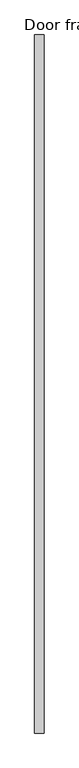
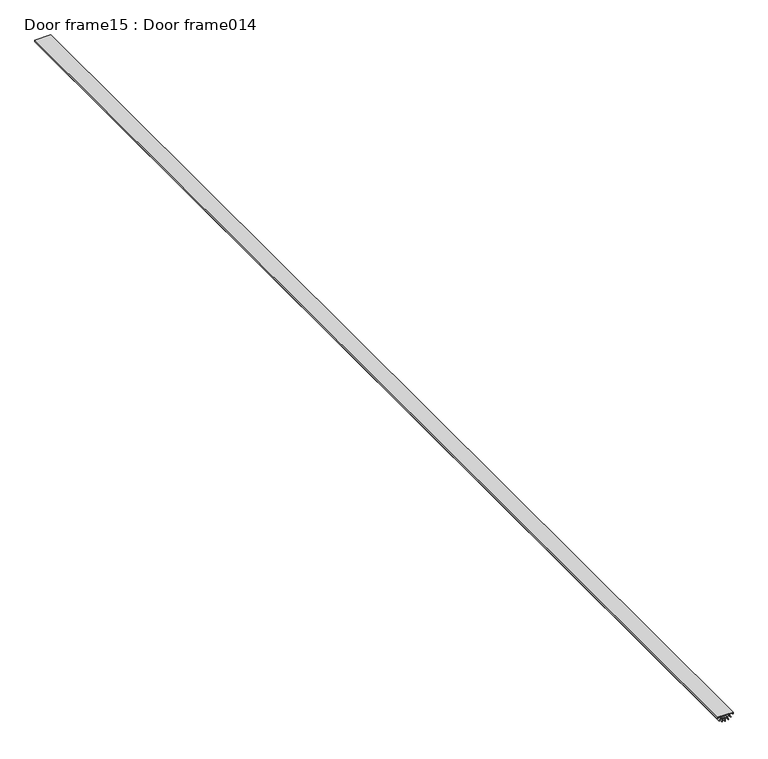
"""IFC4 building model written with IfcOpenShell, lengths in millimetres: proxy geometry, Door frame15 : Door frame014."""

from ifc_helpers import new_model, si_unit, frame, origin, place, context, project, spatial, polyline, outline, extrude, source, transform, mapped, element, save


def door_frame15_door_frame014_1e3dbea9(model_context):
    return source(origin(), model_context, "Body", "SweptSolid", [
        extrude(outline(polyline([(36578.3756733, 15524.8710245), (36578.3756733, 15525.6647745), (36583.8229098, 15525.6647745), (36584.304169, 15528.4194862), (36579.1830903, 15530.2833952), (36579.4545674, 15531.0292768), (36584.573299, 15529.166222), (36585.9800182, 15531.6205482), (36581.8052868, 15535.1235857), (36582.3155014, 15535.731632), (36586.4883159, 15532.2302029), (36588.5541303, 15533.9941318), (36588.5541303, 15536.9862907), (36587.284361, 15536.9862907), (36587.284361, 15538.6848615), (36589.8546103, 15538.6848615), (36589.8546103, 15511.5429442), (36587.284361, 15511.5429442), (36587.284361, 15513.5495083), (36588.5541303, 15513.5495083), (36588.5541303, 15516.5416672), (36586.5323252, 15518.2570371), (36582.3575787, 15514.7540195), (36581.8473669, 15515.362068), (36586.0201974, 15518.8634779), (36584.5980367, 15521.3089171), (36579.4769756, 15519.4449702), (36579.2054928, 15520.1908496), (36584.3242102, 15522.0539435), (36583.8229098, 15524.8710245), (36578.3756733, 15524.8710245)]), holes=[polyline([(36588.5541303, 15532.8858954), (36586.6136518, 15530.8738124), (36585.2069325, 15528.4194862), (36584.7256733, 15525.6647745), (36584.7256733, 15524.8710245), (36585.2269736, 15522.0539435), (36586.6491343, 15519.6085043), (36588.5541303, 15517.6499036), (36588.5541303, 15532.8858954)])]), frame((0.0, -1052.8906567, 0.0), z_axis=(0.0, 1.0, 0.0), x_axis=(0.0, 0.0, 1.0)), (0.0, 0.0, 1.0), 1999.85),
    ])


if __name__ == "__main__":
    model = new_model("IFC4")
    model_context = context("Model", 3, world=origin())
    ifc_project = project(units=[si_unit("LENGTHUNIT", "METRE", prefix="MILLI")], contexts=[model_context])
    site = spatial("IfcSite", under=ifc_project)
    building = spatial("IfcBuilding", under=site)
    placement = place(None, origin())
    door_frame15_door_frame014_shape = door_frame15_door_frame014_1e3dbea9(model_context)
    element("IfcBuildingElementProxy", 1, Name="Door frame15 : Door frame014", ObjectType="Door frame15 : Door frame014", at=placement, inside=building, context=model_context, shape_type="MappedRepresentation", body=[
        mapped(door_frame15_door_frame014_shape, transform((0.0, 0.0, 0.0), x_axis=(1.0, 0.0, 0.0), y_axis=(0.0, 1.0, 0.0), z_axis=(0.0, 0.0, 1.0))),
    ])
    save(model, "model.ifc")

# Revit data of these elements
# Type "Door frame15 : Door frame014"
#   NameOverride = "Door frame014"
# Element 1 (IfcBuildingElementProxy, "Door frame15 : Door frame014")
#   Materials on its faces: "WEATHERSTRIPPING SWEEP"
# Materials
#   "WEATHERSTRIPPING SWEEP": class "Wood", colour RGB 212 179 113, transparency 0, Description = "Plywood, sheathing grade", Cost = 0
